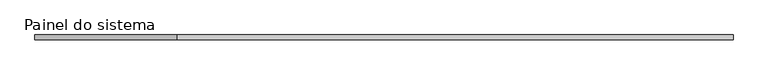
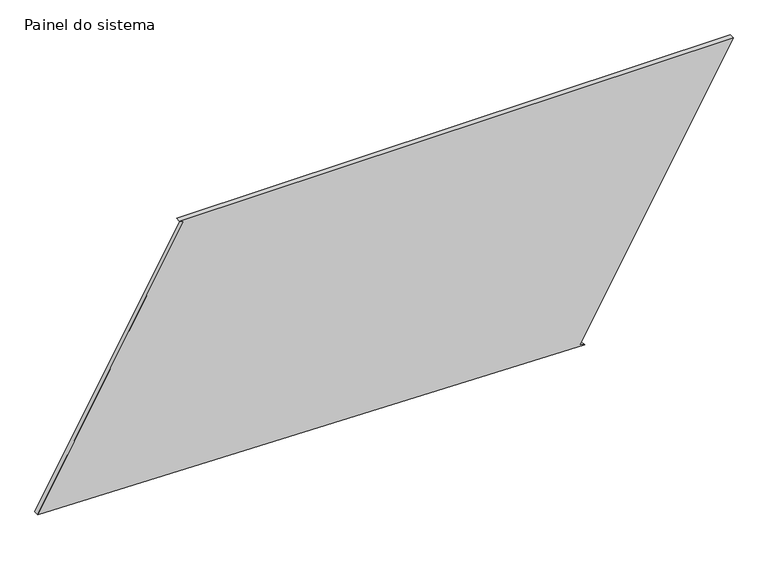
"""IFC4 building model written with IfcOpenShell, lengths in millimetres: plate geometry, Painel do sistema : Envidraçado."""

from ifc_helpers import new_model, si_unit, frame, origin, place, context, project, spatial, polyline, outline, extrude, source, transform, mapped, element, save


def painel_do_sistema_c6ef5303(model_context):
    return source(origin(), model_context, "Body", "SweptSolid", [
        extrude(outline(polyline([(0.0, 1052.2134705), (12.2820845, 1030.4384757), (1441.4768477, 1836.5691346), (1441.4768477, -1088.3786781), (1429.1947631, -1066.6036833), (64.1175532, -1836.5691346), (0.0, 1052.2134705)])), frame((0.0, 24.5, 0.0), z_axis=(0.0, 1.0, 0.0), x_axis=(0.0, 0.0, 1.0)), (0.0, 0.0, 1.0), 25.0),
    ])


if __name__ == "__main__":
    model = new_model("IFC4")
    model_context = context("Model", 3, world=origin())
    ifc_project = project(units=[si_unit("LENGTHUNIT", "METRE", prefix="MILLI")], contexts=[model_context])
    site = spatial("IfcSite", under=ifc_project)
    building = spatial("IfcBuilding", under=site)
    placement = place(None, origin())
    painel_do_sistema_shape = painel_do_sistema_c6ef5303(model_context)
    element("IfcPlate", 1, ObjectType="Painel do sistema : Envidraçado", at=placement, inside=building, context=model_context, shape_type="MappedRepresentation", body=[
        mapped(painel_do_sistema_shape, transform((0.0, 0.0, 0.0), x_axis=(1.0, 0.0, 0.0), y_axis=(0.0, 1.0, 0.0), z_axis=(0.0, 0.0, 1.0))),
    ])
    save(model, "model.ifc")

# Revit data of these elements
# Type "Painel do sistema : Envidraçado"
#   Construction Type Id = "GSP4R"
#   Analytic Construction = "Vidraça única Pilkington 1/8 pol"
#   Visual Light Transmittance = 0.9
#   Solar Heat Gain Coefficient = 0.86
#   Heat Transfer Coefficient (U) = 6.7069 W/(m²·K)
# Element 1 (IfcPlate, "Painel do sistema : Envidraçado")
#   Materials on its faces: "Vidro"
# Materials
#   "Vidro": class "Vidro", colour RGB 0 128 192, transparency 0.9, Description = "Vidro de sílica", Cost = 0
